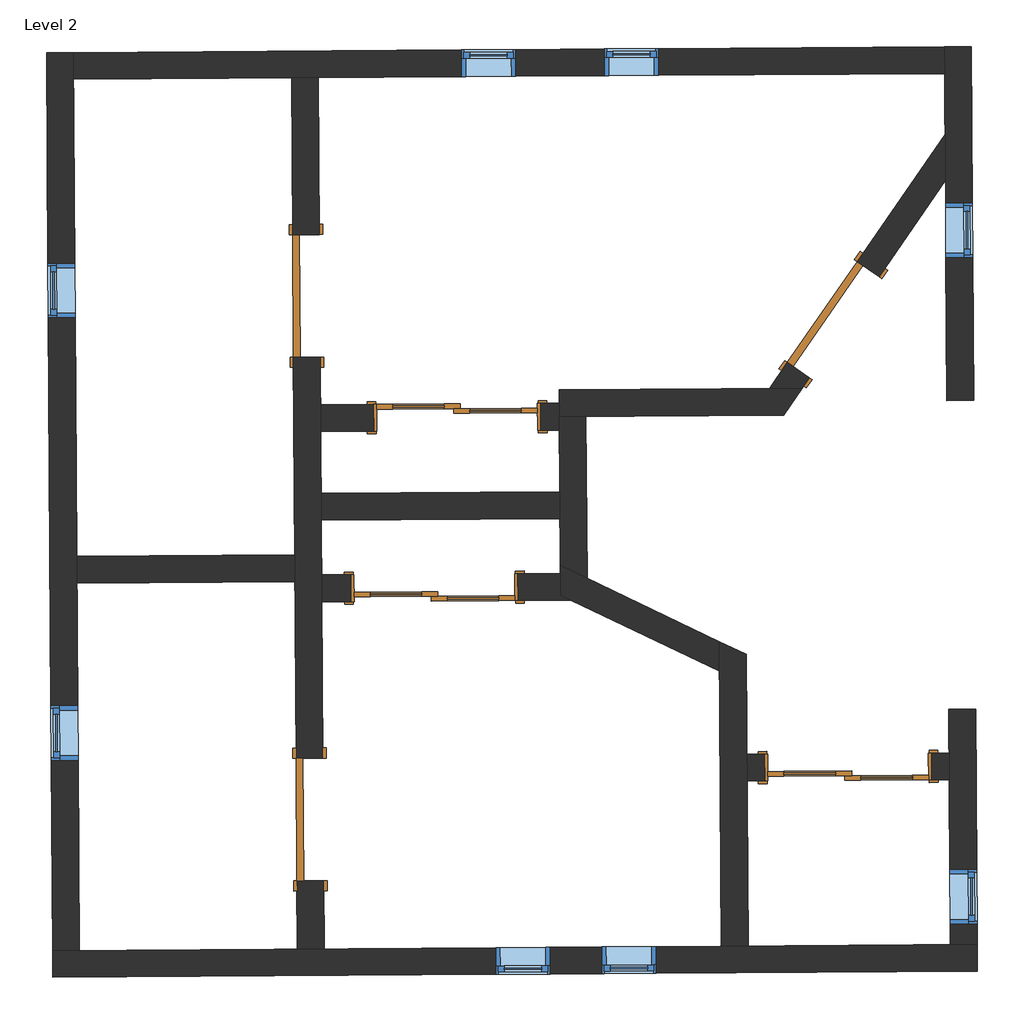
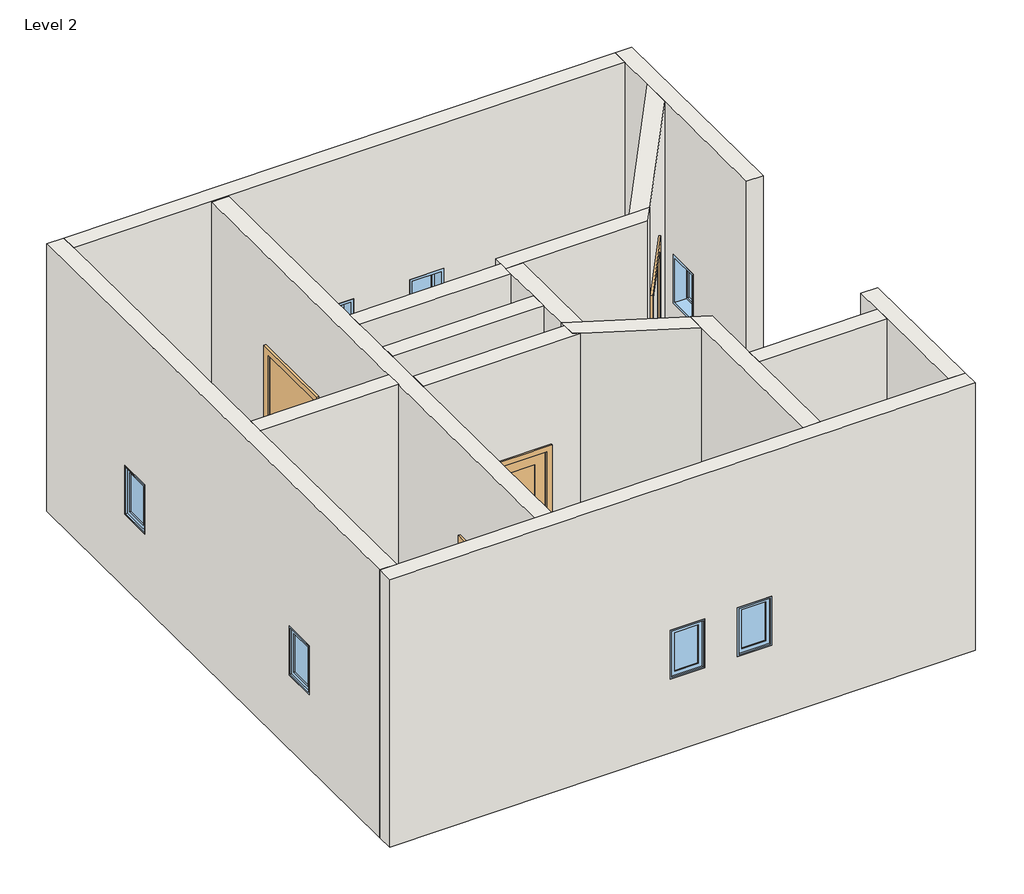
# One storey: 16 walls, 8 windows, 6 doors.
"""IFC4 building model written with IfcOpenShell, lengths in millimetres."""

import ifcopenshell
import ifcopenshell.guid

model = None  # the IFC model being written
_history = None  # IfcOwnerHistory: only IFC2X3 demands one
_inside = {}  # id of a spatial element -> (the spatial element, [elements in it])
_under = {}  # id of a project, library or spatial element -> (it, [spatial elements below it])
_declared = {}  # id of a project -> (the project, [libraries it declares])
_typed = {}  # id of a type object -> (the type object, [elements of that type])
_made_of = {}  # id of a material, layer set ... -> (it, [elements and type objects made of it])


def new_model(schema):
    """Start an empty IFC model of exactly this schema.

    Asked for "IFC4X3", IfcOpenShell would pick the latest addendum, in which some entities
    have other attributes; the version numbers below select the first issue.
    IFC2X3 requires an IfcOwnerHistory on every rooted entity: one is made here for all.
    """
    global model, _history
    if schema == "IFC4X3":
        model = ifcopenshell.file(schema_version=(4, 3, 0, 0))
    else:
        model = ifcopenshell.file(schema=schema)
    _inside.clear()
    _under.clear()
    _declared.clear()
    _typed.clear()
    _made_of.clear()
    _history = None
    if model.schema == "IFC2X3":
        org = make("IfcOrganization", Name="unknown")
        user = make(
            "IfcPersonAndOrganization",
            ThePerson=make("IfcPerson", FamilyName="unknown"),
            TheOrganization=org,
        )
        app = make(
            "IfcApplication",
            ApplicationDeveloper=org,
            Version="unknown",
            ApplicationFullName="unknown",
            ApplicationIdentifier="unknown",
        )
        _history = make(
            "IfcOwnerHistory",
            OwningUser=user,
            OwningApplication=app,
            ChangeAction="ADDED",
            CreationDate=0,
        )
    return model


def make(cls, **values):
    """One entity of the class cls with the attributes given. An attribute that is None is left unset."""
    return model.create_entity(
        cls, **{name: value for name, value in values.items() if value is not None}
    )


def rooted(cls, **values):
    """An entity with a GlobalId (a new one), such as an element, a storey or a relation."""
    return make(cls, GlobalId=ifcopenshell.guid.new(), OwnerHistory=_history, **values)


def si_unit(unit_type, name, prefix=None):
    """IfcSIUnit, for example si_unit("LENGTHUNIT", "METRE", prefix="MILLI")."""
    return make("IfcSIUnit", UnitType=unit_type, Prefix=prefix, Name=name)


def assignment(units):
    """IfcUnitAssignment: the units of a project."""
    return None if units is None else make("IfcUnitAssignment", Units=units)


def point(xyz):
    """IfcCartesianPoint."""
    return None if xyz is None else make("IfcCartesianPoint", Coordinates=xyz)


def direction(xyz):
    """IfcDirection."""
    return None if xyz is None else make("IfcDirection", DirectionRatios=xyz)


def frame(location, z_axis=None, x_axis=None):
    """IfcAxis2Placement3D, a coordinate frame: its origin and axes. An axis left out is left unset."""
    return make(
        "IfcAxis2Placement3D",
        Location=point(location),
        Axis=direction(z_axis),
        RefDirection=direction(x_axis),
    )


def origin():
    """The frame at (0, 0, 0) with its axes left unset."""
    return frame((0.0, 0.0, 0.0))


def origin_with_axes():
    """The frame at (0, 0, 0) with the z axis (0, 0, 1) and the x axis (1, 0, 0) written out."""
    return frame((0.0, 0.0, 0.0), z_axis=(0.0, 0.0, 1.0), x_axis=(1.0, 0.0, 0.0))


def place(relative_to, where):
    """IfcLocalPlacement: puts the frame where relative to a parent placement (None: the world)."""
    return make(
        "IfcLocalPlacement", PlacementRelTo=relative_to, RelativePlacement=where
    )


def context(
    kind, dimensions, precision=None, world=None, true_north=None, identifier=None
):
    """IfcGeometricRepresentationContext, for example the 3D "Model" context."""
    return make(
        "IfcGeometricRepresentationContext",
        ContextIdentifier=identifier,
        ContextType=kind,
        CoordinateSpaceDimension=dimensions,
        Precision=precision,
        WorldCoordinateSystem=world,
        TrueNorth=true_north,
    )


def project(units=None, contexts=None):
    """IfcProject with its units and contexts."""
    return rooted(
        "IfcProject",
        Name="project",
        RepresentationContexts=contexts,
        UnitsInContext=assignment(units),
    )


def spatial(cls, under=None, at=None, **own):
    """A site, building, storey or space (cls), placed at a placement, below another one or the project."""
    s = rooted(cls, ObjectPlacement=at, **own)
    if under is not None:
        _under.setdefault(under.id(), (under, []))[1].append(s)
    return s


def polyline(points):
    """IfcPolyline through the points."""
    return make("IfcPolyline", Points=[point(p) for p in points])


def outline(outer, holes=None, kind="AREA"):
    """IfcArbitraryClosedProfileDef: a profile drawn as a closed curve; with holes, ...WithVoids."""
    if holes is None:
        return make("IfcArbitraryClosedProfileDef", ProfileType=kind, OuterCurve=outer)
    return make(
        "IfcArbitraryProfileDefWithVoids",
        ProfileType=kind,
        OuterCurve=outer,
        InnerCurves=holes,
    )


def extrude(swept, where, along, depth):
    """IfcExtrudedAreaSolid: the profile swept, set in the frame where, extruded along a direction by depth."""
    return make(
        "IfcExtrudedAreaSolid",
        SweptArea=swept,
        Position=where,
        ExtrudedDirection=direction(along),
        Depth=depth,
    )


def faces_of(points, faces, orient=None, outer=None):
    """IfcFace entities. A face is a list of loops; a loop is a list of indices into points, from 0.

    orient and outer hold one flag for each loop. By default every Orientation is true, the
    first loop of a face is its IfcFaceOuterBound and the others are IfcFaceBound.
    """
    made = []
    for i, loops in enumerate(faces):
        bounds = []
        for j, loop in enumerate(loops):
            is_outer = j == 0 if outer is None else outer[i][j]
            bounds.append(
                make(
                    "IfcFaceOuterBound" if is_outer else "IfcFaceBound",
                    Bound=make("IfcPolyLoop", Polygon=[points[k] for k in loop]),
                    Orientation=True if orient is None else orient[i][j],
                )
            )
        made.append(make("IfcFace", Bounds=bounds))
    return made


def faceted_brep(points, faces, orient=None, outer=None, voids=None):
    """IfcFacetedBrep: a solid bounded by flat faces; with voids (closed shells), ...WithVoids."""
    shared = [point(p) for p in points]
    hull = make("IfcClosedShell", CfsFaces=faces_of(shared, faces, orient, outer))
    if voids is None:
        return make("IfcFacetedBrep", Outer=hull)
    return make(
        "IfcFacetedBrepWithVoids",
        Outer=hull,
        Voids=[
            make(cls, CfsFaces=faces_of(shared, fs, o, b)) for cls, fs, o, b in voids
        ],
    )


def shape(context_of_items, identifier, shape_type, items):
    """IfcShapeRepresentation: the items that make up one representation, for example the "Body"."""
    return make(
        "IfcShapeRepresentation",
        ContextOfItems=context_of_items,
        RepresentationIdentifier=identifier,
        RepresentationType=shape_type,
        Items=items,
    )


def source(mapping_origin, context_of_items, identifier, shape_type, items):
    """IfcRepresentationMap: a shape defined once, which mapped items show again and again."""
    return make(
        "IfcRepresentationMap",
        MappingOrigin=mapping_origin,
        MappedRepresentation=shape(context_of_items, identifier, shape_type, items),
    )


def transform(
    local_origin,
    x_axis=None,
    y_axis=None,
    z_axis=None,
    scale=None,
    scale2=None,
    scale3=None,
    uniform=True,
):
    """IfcCartesianTransformationOperator3D, or its non-uniform kind. x_axis, y_axis, z_axis: its Axis1, 2, 3."""
    if uniform:
        return make(
            "IfcCartesianTransformationOperator3D",
            Axis1=direction(x_axis),
            Axis2=direction(y_axis),
            LocalOrigin=point(local_origin),
            Scale=scale,
            Axis3=direction(z_axis),
        )
    return make(
        "IfcCartesianTransformationOperator3DnonUniform",
        Axis1=direction(x_axis),
        Axis2=direction(y_axis),
        LocalOrigin=point(local_origin),
        Scale=scale,
        Axis3=direction(z_axis),
        Scale2=scale2,
        Scale3=scale3,
    )


def mapped(mapping_source, mapping_target):
    """IfcMappedItem: shows the shape of a source again, moved by a transform."""
    return make(
        "IfcMappedItem", MappingSource=mapping_source, MappingTarget=mapping_target
    )


def made_of(thing, what):
    """Note that an element or type object is made of a material, layer set ...; save() writes the relation."""
    if what is not None:
        _made_of.setdefault(what.id(), (what, []))[1].append(thing)
    return thing


def element(
    cls,
    number,
    at=None,
    inside=None,
    cuts=None,
    type_object=None,
    material=None,
    context=None,
    identifier="Body",
    shape_type=None,
    held_by="IfcProductDefinitionShape",
    body=None,
    shapes=None,
    **own,
):
    """One element of the class cls, such as IfcWall. Its Tag is "e" and its number.

    at: its placement. inside: the storey or other place that contains it. cuts: it is an
    opening in that element (IfcRelVoidsElement). A single representation is given by context,
    identifier, shape_type and body (its items); several are given by shapes. held_by: the class
    of the entity that holds the representations. save() writes the other relations.
    """
    e = rooted(cls, Tag="e%d" % number, ObjectPlacement=at, **own)
    if body is not None:
        shapes = [shape(context, identifier, shape_type, body)]
    if shapes is not None:
        e.Representation = make(held_by, Representations=shapes)
    if inside is not None:
        _inside.setdefault(inside.id(), (inside, []))[1].append(e)
    if cuts is not None:
        rooted(
            "IfcRelVoidsElement", RelatingBuildingElement=cuts, RelatedOpeningElement=e
        )
    if type_object is not None:
        _typed.setdefault(type_object.id(), (type_object, []))[1].append(e)
    return made_of(e, material)


def aggregate(whole, parts):
    """IfcRelAggregates: a whole, such as a stair, and the parts it consists of."""
    return rooted("IfcRelAggregates", RelatingObject=whole, RelatedObjects=parts)


def save(model, path):
    """Write the relations noted so far, then the file.

    IfcRelAggregates (storeys below a building ...), IfcRelContainedInSpatialStructure (elements
    in a storey), IfcRelDefinesByType, IfcRelAssociatesMaterial and IfcRelDeclares: one each for
    every whole, place, type object, material and project.
    """
    for whole, parts in _under.values():
        aggregate(whole, parts)
    for where, things in _inside.values():
        rooted(
            "IfcRelContainedInSpatialStructure",
            RelatedElements=things,
            RelatingStructure=where,
        )
    for kind, things in _typed.values():
        rooted("IfcRelDefinesByType", RelatedObjects=things, RelatingType=kind)
    for what, things in _made_of.values():
        rooted("IfcRelAssociatesMaterial", RelatedObjects=things, RelatingMaterial=what)
    for by, libraries in _declared.values():
        rooted("IfcRelDeclares", RelatingContext=by, RelatedDefinitions=libraries)
    model.write(path)


def m_door_interior_double_sliding_2_panel_wood_1200_x_2000mm_2523b4d6(model_context):
    return source(origin(), model_context, "Body", "SweptSolid", [
        extrude(outline(polyline([(480.0, 38.4916667), (94.6, 38.4916667), (94.6, 50.1583333), (480.0, 50.1583333), (480.0, 38.4916667)])), frame((0.0, 0.0, 1014.4), z_axis=(0.0, 0.0, 1.0), x_axis=(1.0, 0.0, 0.0)), (0.0, 0.0, 1.0), 865.6),
        extrude(outline(polyline([(480.0, 38.4916667), (94.6, 38.4916667), (94.6, 50.1583333), (480.0, 50.1583333), (480.0, 38.4916667)])), frame((0.0, 0.0, 230.0), z_axis=(0.0, 0.0, 1.0), x_axis=(1.0, 0.0, 0.0)), (0.0, 0.0, 1.0), 584.4),
        extrude(outline(polyline([(2000.0, -25.4), (0.0, -25.4), (0.0, 600.0), (2000.0, 600.0), (2000.0, -25.4)]), holes=[polyline([(1880.0, 94.6), (1880.0, 480.0), (1014.4, 480.0), (1014.4, 94.6), (1880.0, 94.6)]), polyline([(814.4, 94.6), (814.4, 480.0), (230.0, 480.0), (230.0, 94.6), (814.4, 94.6)])]), frame((0.0, 26.825, 0.0), z_axis=(0.0, 1.0, 0.0), x_axis=(0.0, 0.0, 1.0)), (0.0, 0.0, 1.0), 35.0),
        extrude(outline(polyline([(-94.6, 73.4916667), (-480.0, 73.4916667), (-480.0, 85.1583333), (-94.6, 85.1583333), (-94.6, 73.4916667)])), frame((0.0, 0.0, 1014.4), z_axis=(0.0, 0.0, 1.0), x_axis=(1.0, 0.0, 0.0)), (0.0, 0.0, 1.0), 865.6),
        extrude(outline(polyline([(-94.6, 73.4916667), (-480.0, 73.4916667), (-480.0, 85.1583333), (-94.6, 85.1583333), (-94.6, 73.4916667)])), frame((0.0, 0.0, 230.0), z_axis=(0.0, 0.0, 1.0), x_axis=(1.0, 0.0, 0.0)), (0.0, 0.0, 1.0), 584.4),
        extrude(outline(polyline([(2000.0, -600.0), (0.0, -600.0), (0.0, 25.4), (2000.0, 25.4), (2000.0, -600.0)]), holes=[polyline([(1880.0, -480.0), (1880.0, -94.6), (1014.4, -94.6), (1014.4, -480.0), (1880.0, -480.0)]), polyline([(814.4, -480.0), (814.4, -94.6), (230.0, -94.6), (230.0, -480.0), (814.4, -480.0)])]), frame((0.0, 61.825, 0.0), z_axis=(0.0, 1.0, 0.0), x_axis=(0.0, 0.0, 1.0)), (0.0, 0.0, 1.0), 35.0),
        extrude(outline(polyline([(0.0, 600.0), (0.0, 625.0), (2025.0, 625.0), (2025.0, -625.0), (0.0, -625.0), (0.0, -600.0), (2000.0, -600.0), (2000.0, 600.0), (0.0, 600.0)])), frame((0.0, -103.175, 0.0), z_axis=(0.0, 1.0, 0.0), x_axis=(0.0, 0.0, 1.0)), (0.0, 0.0, 1.0), 200.0),
        extrude(outline(polyline([(0.0, 606.35), (0.0, 671.35), (2071.35, 671.35), (2071.35, -671.35), (0.0, -671.35), (0.0, -606.35), (2006.35, -606.35), (2006.35, 606.35), (0.0, 606.35)])), frame((0.0, -123.175, 0.0), z_axis=(0.0, 1.0, 0.0), x_axis=(0.0, 0.0, 1.0)), (0.0, 0.0, 1.0), 20.0),
        extrude(outline(polyline([(0.0, 606.35), (0.0, 671.35), (2071.35, 671.35), (2071.35, -671.35), (0.0, -671.35), (0.0, -606.35), (2006.35, -606.35), (2006.35, 606.35), (0.0, 606.35)])), frame((0.0, 96.825, 0.0), z_axis=(0.0, 1.0, 0.0), x_axis=(0.0, 0.0, 1.0)), (0.0, 0.0, 1.0), 20.0),
    ])


def m_single_flush_0915_x_2134mm_6a9e8738(model_context):
    return source(origin(), model_context, "Body", "SweptSolid", [
        extrude(outline(polyline([(2210.0, -533.5), (0.0, -533.5), (0.0, -457.5), (2134.0, -457.5), (2134.0, 457.5), (0.0, 457.5), (0.0, 533.5), (2210.0, 533.5), (2210.0, -533.5)])), frame((0.0, 100.0, 0.0), z_axis=(0.0, 1.0, 0.0), x_axis=(0.0, 0.0, 1.0)), (0.0, 0.0, 1.0), 25.0),
        extrude(outline(polyline([(2210.0, 533.5), (2210.0, -533.5), (0.0, -533.5), (0.0, -457.5), (2134.0, -457.5), (2134.0, 457.5), (0.0, 457.5), (0.0, 533.5), (2210.0, 533.5)])), frame((0.0, -125.0, 0.0), z_axis=(0.0, 1.0, 0.0), x_axis=(0.0, 0.0, 1.0)), (0.0, 0.0, 1.0), 25.0),
        extrude(outline(polyline([(457.5, 49.0), (-457.5, 49.0), (-457.5, 100.0), (457.5, 100.0), (457.5, 49.0)])), origin_with_axes(), (0.0, 0.0, 1.0), 2134.0),
    ])


def m_single_flush_0915_x_2134mm_727434cd(model_context):
    return source(origin(), model_context, "Body", "SweptSolid", [
        extrude(outline(polyline([(2210.0, -533.5), (0.0, -533.5), (0.0, -457.5), (2134.0, -457.5), (2134.0, 457.5), (0.0, 457.5), (0.0, 533.5), (2210.0, 533.5), (2210.0, -533.5)])), frame((0.0, -125.0, 0.0), z_axis=(0.0, 1.0, 0.0), x_axis=(0.0, 0.0, 1.0)), (0.0, 0.0, 1.0), 25.0),
        extrude(outline(polyline([(2210.0, 533.5), (2210.0, -533.5), (0.0, -533.5), (0.0, -457.5), (2134.0, -457.5), (2134.0, 457.5), (0.0, 457.5), (0.0, 533.5), (2210.0, 533.5)])), frame((0.0, 100.0, 0.0), z_axis=(0.0, 1.0, 0.0), x_axis=(0.0, 0.0, 1.0)), (0.0, 0.0, 1.0), 25.0),
        extrude(outline(polyline([(457.5, -49.0), (457.5, -100.0), (-457.5, -100.0), (-457.5, -49.0), (457.5, -49.0)])), origin_with_axes(), (0.0, 0.0, 1.0), 2134.0),
    ])


def m_fixed_0406_x_0610mm_8205b201(model_context):
    return source(origin(), model_context, "Body", "SweptSolid", [
        extrude(outline(polyline([(-140.0, 78.0), (140.0, 78.0), (140.0, 66.0), (-140.0, 66.0), (-140.0, 78.0)])), frame((0.0, 0.0, 978.0), z_axis=(0.0, 0.0, 1.0), x_axis=(1.0, 0.0, 0.0)), (0.0, 0.0, 1.0), 484.0),
        extrude(outline(polyline([(1506.0, -184.0), (934.0, -184.0), (934.0, 184.0), (1506.0, 184.0), (1506.0, -184.0)]), holes=[polyline([(1462.0, -140.0), (1462.0, 140.0), (978.0, 140.0), (978.0, -140.0), (1462.0, -140.0)])]), frame((0.0, 50.0, 0.0), z_axis=(0.0, 1.0, 0.0), x_axis=(0.0, 0.0, 1.0)), (0.0, 0.0, 1.0), 44.0),
        extrude(outline(polyline([(1525.0, -203.0), (915.0, -203.0), (915.0, 203.0), (1525.0, 203.0), (1525.0, -203.0)]), holes=[polyline([(1506.0, -184.0), (1506.0, 184.0), (934.0, 184.0), (934.0, -184.0), (1506.0, -184.0)])]), frame((0.0, 50.0, 0.0), z_axis=(0.0, 1.0, 0.0), x_axis=(0.0, 0.0, 1.0)), (0.0, 0.0, 1.0), 63.0),
        extrude(outline(polyline([(1525.0, -203.0), (915.0, -203.0), (915.0, 203.0), (1525.0, 203.0), (1525.0, -203.0)]), holes=[polyline([(1493.0, -171.0), (1493.0, 171.0), (947.0, 171.0), (947.0, -171.0), (1493.0, -171.0)])]), frame((0.0, -87.0, 0.0), z_axis=(0.0, 1.0, 0.0), x_axis=(0.0, 0.0, 1.0)), (0.0, 0.0, 1.0), 137.0),
    ])


model = new_model("IFC4")

# Units and contexts
model_context = context("Model", 3, world=origin())
ifc_project = project(units=[si_unit("LENGTHUNIT", "METRE", prefix="MILLI")], contexts=[model_context])

# Site, building, storey
site = spatial("IfcSite", under=ifc_project)
building = spatial("IfcBuilding", under=site)
storey = spatial("IfcBuildingStorey", under=building, Name="Level 2", Elevation=3048.0)

# Doors
placement = place(None, origin())
m_door_interior_double_sliding_2_panel_wood_1200_x_2000mm_shape = m_door_interior_double_sliding_2_panel_wood_1200_x_2000mm_2523b4d6(model_context)
element("IfcDoor", 1, ObjectType="M_Door-Interior-Double-Sliding-2_Panel-Wood : 1200 x 2000mm", at=placement, inside=storey, context=model_context, shape_type="MappedRepresentation", body=[
    mapped(m_door_interior_double_sliding_2_panel_wood_1200_x_2000mm_shape, transform((-71556.4861073, -7431.0700017, 3048.0), x_axis=(0.9999777944135733, 0.006664133834601911, 0.0), y_axis=(-0.006664133834601911, 0.9999777944135733, 0.0), z_axis=(0.0, 0.0, 1.0))),
])
element("IfcDoor", 2, ObjectType="M_Door-Interior-Double-Sliding-2_Panel-Wood : 1200 x 2000mm", at=placement, inside=storey, context=model_context, shape_type="MappedRepresentation", body=[
    mapped(m_door_interior_double_sliding_2_panel_wood_1200_x_2000mm_shape, transform((-71726.571382, -8709.3309667, 3048.0), x_axis=(-0.9999777944135733, -0.006664133834601911, 0.0), y_axis=(0.006664133834601911, -0.9999777944135733, 0.0), z_axis=(0.0, 0.0, 1.0))),
])
element("IfcDoor", 3, ObjectType="M_Door-Interior-Double-Sliding-2_Panel-Wood : 1200 x 2000mm", at=placement, inside=storey, context=model_context, shape_type="MappedRepresentation", body=[
    mapped(m_door_interior_double_sliding_2_panel_wood_1200_x_2000mm_shape, transform((-68636.4800539, -10048.7108484, 3048.0), x_axis=(-0.9999777944135733, -0.006664133834601911, 0.0), y_axis=(0.006664133834601911, -0.9999777944135733, 0.0), z_axis=(0.0, 0.0, 1.0))),
])
m_single_flush_0915_x_2134mm_shape = m_single_flush_0915_x_2134mm_6a9e8738(model_context)
element("IfcDoor", 4, ObjectType="M_Single-Flush : 0915 x 2134mm", at=placement, inside=storey, context=model_context, shape_type="MappedRepresentation", body=[
    mapped(m_single_flush_0915_x_2134mm_shape, transform((-68747.95097, -6705.2508945, 3048.0), x_axis=(0.5681047608958888, 0.8229562446736918, 0.0), y_axis=(-0.8229562446736918, 0.5681047608958888, 0.0), z_axis=(0.0, 0.0, 1.0))),
])
element("IfcDoor", 5, ObjectType="M_Single-Flush : 0915 x 2134mm", at=placement, inside=storey, context=model_context, shape_type="MappedRepresentation", body=[
    mapped(m_single_flush_0915_x_2134mm_shape, transform((-72681.7331306, -6527.4212039, 3048.0), x_axis=(-0.0066641338345986775, 0.9999777944135734, 0.0), y_axis=(-0.9999777944135734, -0.0066641338345986775, 0.0), z_axis=(0.0, 0.0, 1.0))),
])
m_single_flush_0915_x_2134mm_2_shape = m_single_flush_0915_x_2134mm_727434cd(model_context)
element("IfcDoor", 6, ObjectType="M_Single-Flush : 0915 x 2134mm", at=placement, inside=storey, context=model_context, shape_type="MappedRepresentation", body=[
    mapped(m_single_flush_0915_x_2134mm_2_shape, transform((-72655.6757177, -10437.4318493, 3048.0), x_axis=(0.0066641338345986775, -0.9999777944135734, 0.0), y_axis=(0.9999777944135734, 0.0066641338345986775, 0.0), z_axis=(0.0, 0.0, 1.0))),
])

# Walls
element("IfcWall", 7, ObjectType="Generic - 200mm", at=placement, inside=storey, context=model_context, shape_type="Brep", body=[
    faceted_brep([(-67672.5433459, -11371.0443197, 3048.0), (-67872.5389048, -11372.3771465, 3048.0), (-69382.7115618, -11382.4413627, 3048.0), (-69582.7071207, -11383.7741894, 3048.0), (-72549.2350537, -11403.5439676, 3048.0), (-72749.2306126, -11404.8767944, 3048.0), (-74377.9944441, -11415.7313355, 3048.0), (-74577.990003, -11417.0641623, 3048.0), (-74577.990003, -11417.0641623, 6372.225), (-74377.9944441, -11415.7313355, 6372.225), (-69582.7071207, -11383.7741894, 6372.225), (-69382.7115618, -11382.4413627, 6372.225), (-67872.5389048, -11372.3771465, 6372.225), (-67672.5433459, -11371.0443197, 6372.225), (-70862.9755949, -11392.3062593, 3963.0), (-70862.9755949, -11392.3062593, 4573.0), (-71268.9665794, -11395.0118977, 4573.0), (-71268.9665794, -11395.0118977, 3963.0), (-70071.3447219, -11387.0306081, 3963.0), (-70071.3447219, -11387.0306081, 4573.0), (-70477.3357065, -11389.7362464, 4573.0), (-70477.3357065, -11389.7362464, 3963.0), (-67671.2105191, -11571.0398786, 3048.0), (-67671.2105191, -11571.0398786, 6372.225), (-74576.6571762, -11617.0597212, 6372.225), (-74576.6571762, -11617.0597212, 3048.0), (-70861.6427681, -11592.3018182, 3963.0), (-71267.6337527, -11595.0074566, 3963.0), (-71267.6337527, -11595.0074566, 4573.0), (-70861.6427681, -11592.3018182, 4573.0), (-70070.0118952, -11587.026167, 3963.0), (-70476.0028797, -11589.7318053, 3963.0), (-70476.0028797, -11589.7318053, 4573.0), (-70070.0118952, -11587.026167, 4573.0)], [[[0, 1, 2, 3, 4, 5, 6, 7, 8, 9, 10, 11, 12, 13], [14, 15, 16, 17], [18, 19, 20, 21]], [[22, 23, 24, 25], [26, 27, 28, 29], [30, 31, 32, 33]], [[7, 6, 5, 4, 3, 2, 1, 0, 22, 25]], [[13, 12, 11, 10, 9, 8, 24, 23]], [[8, 7, 25, 24]], [[0, 13, 23, 22]], [[15, 14, 26, 29]], [[16, 15, 29, 28]], [[17, 16, 28, 27]], [[14, 17, 27, 26]], [[19, 18, 30, 33]], [[20, 19, 33, 32]], [[21, 20, 32, 31]], [[18, 21, 31, 30]]]),
])
element("IfcWall", 8, ObjectType="Generic - 200mm", at=placement, inside=storey, context=model_context, shape_type="Brep", body=[
    faceted_brep([(-74377.9944441, -11415.7313355, 3048.0), (-74396.2767952, -8672.3973113, 3048.0), (-74397.6096219, -8472.4017524, 3048.0), (-74421.3486332, -4910.2757962, 3048.0), (-74422.6814599, -4710.2802373, 3048.0), (-74422.6814599, -4710.2802373, 6372.225), (-74421.3486332, -4910.2757962, 6372.225), (-74397.6096219, -8472.4017524, 6372.225), (-74396.2767952, -8672.3973113, 6372.225), (-74377.9944441, -11415.7313355, 6372.225), (-74409.4904734, -6689.6362836, 3963.0), (-74409.4904734, -6689.6362836, 4573.0), (-74412.1961118, -6283.6452991, 4573.0), (-74412.1961118, -6283.6452991, 3963.0), (-74387.4654774, -9994.567951, 3963.0), (-74387.4654774, -9994.567951, 4573.0), (-74390.1711157, -9588.5769665, 4573.0), (-74390.1711157, -9588.5769665, 3963.0), (-74577.990003, -11417.0641623, 3048.0), (-74577.990003, -11417.0641623, 6372.225), (-74622.6770188, -4711.6130641, 6372.225), (-74622.6770188, -4711.6130641, 3048.0), (-74609.4860323, -6690.9691104, 3963.0), (-74612.1916706, -6284.9781258, 3963.0), (-74612.1916706, -6284.9781258, 4573.0), (-74609.4860323, -6690.9691104, 4573.0), (-74587.4610363, -9995.9007778, 3963.0), (-74590.1666746, -9589.9097933, 3963.0), (-74590.1666746, -9589.9097933, 4573.0), (-74587.4610363, -9995.9007778, 4573.0)], [[[0, 1, 2, 3, 4, 5, 6, 7, 8, 9], [10, 11, 12, 13], [14, 15, 16, 17]], [[18, 19, 20, 21], [22, 23, 24, 25], [26, 27, 28, 29]], [[4, 3, 2, 1, 0, 18, 21]], [[9, 8, 7, 6, 5, 20, 19]], [[0, 9, 19, 18]], [[5, 4, 21, 20]], [[11, 10, 22, 25]], [[12, 11, 25, 24]], [[13, 12, 24, 23]], [[10, 13, 23, 22]], [[15, 14, 26, 29]], [[16, 15, 29, 28]], [[17, 16, 28, 27]], [[14, 17, 27, 26]]]),
])
element("IfcWall", 9, ObjectType="Generic - 200mm", at=placement, inside=storey, context=model_context, shape_type="Brep", body=[
    faceted_brep([(-74421.3486332, -4910.2757962, 3048.0), (-72792.5848016, -4899.421255, 3048.0), (-72592.5892428, -4898.0884283, 3048.0), (-67915.8930938, -4866.9216071, 3048.0), (-67915.8930938, -4866.9216071, 6372.225), (-74421.3486332, -4910.2757962, 6372.225), (-70457.2366606, -4883.8578369, 3963.0), (-70457.2366606, -4883.8578369, 4573.0), (-70051.245676, -4881.1521985, 4573.0), (-70051.245676, -4881.1521985, 3963.0), (-71524.0129716, -4890.9671348, 3963.0), (-71524.0129716, -4890.9671348, 4573.0), (-71118.0219871, -4888.2614965, 4573.0), (-71118.0219871, -4888.2614965, 3963.0), (-74422.6814599, -4710.2802373, 3048.0), (-74422.6814599, -4710.2802373, 6372.225), (-67917.2259206, -4666.9260483, 6372.225), (-67917.2259206, -4666.9260483, 3048.0), (-70458.5694873, -4683.862278, 3963.0), (-70052.5785028, -4681.1566396, 3963.0), (-70052.5785028, -4681.1566396, 4573.0), (-70458.5694873, -4683.862278, 4573.0), (-71525.3457984, -4690.971576, 3963.0), (-71119.3548139, -4688.2659376, 3963.0), (-71119.3548139, -4688.2659376, 4573.0), (-71525.3457984, -4690.971576, 4573.0)], [[[0, 1, 2, 3, 4, 5], [6, 7, 8, 9], [10, 11, 12, 13]], [[14, 15, 16, 17], [18, 19, 20, 21], [22, 23, 24, 25]], [[3, 2, 1, 0, 14, 17]], [[5, 4, 16, 15]], [[0, 5, 15, 14]], [[7, 6, 18, 21]], [[8, 7, 21, 20]], [[9, 8, 20, 19]], [[6, 9, 19, 18]], [[11, 10, 22, 25]], [[12, 11, 25, 24]], [[13, 12, 24, 23]], [[10, 13, 23, 22]], [[4, 3, 17, 16]]]),
])
element("IfcWall", 10, ObjectType="Generic - 200mm", at=placement, inside=storey, context=model_context, shape_type="Brep", body=[
    faceted_brep([(-67917.2259206, -4666.9260483, 3048.0), (-67915.8930938, -4866.9216071, 3048.0), (-67912.8767245, -5319.5389284, 3048.0), (-67910.5530119, -5668.2205446, 3048.0), (-67899.6125812, -7309.8724158, 3048.0), (-67899.6125812, -7309.8724158, 6372.225), (-67910.5530119, -5668.2205446, 6372.225), (-67912.8767245, -5319.5389284, 6372.225), (-67915.8930938, -4866.9216071, 6372.225), (-67917.2259206, -4666.9260483, 6372.225), (-67909.4388634, -5835.4026295, 3963.0), (-67909.4388634, -5835.4026295, 4573.0), (-67906.733225, -6241.393614, 4573.0), (-67906.733225, -6241.393614, 3963.0), (-67717.2303617, -4665.5932215, 3048.0), (-67717.2303617, -4665.5932215, 6372.225), (-67699.6170223, -7308.539589, 6372.225), (-67699.6170223, -7308.539589, 3048.0), (-67709.4433045, -5834.0698027, 3963.0), (-67706.7376661, -6240.0607872, 3963.0), (-67706.7376661, -6240.0607872, 4573.0), (-67709.4433045, -5834.0698027, 4573.0)], [[[0, 1, 2, 3, 4, 5, 6, 7, 8, 9], [10, 11, 12, 13]], [[14, 15, 16, 17], [18, 19, 20, 21]], [[4, 3, 2, 1, 0, 14, 17]], [[5, 4, 17, 16]], [[9, 8, 7, 6, 5, 16, 15]], [[11, 10, 18, 21]], [[12, 11, 21, 20]], [[13, 12, 20, 19]], [[10, 13, 19, 18]], [[0, 9, 15, 14]]]),
])
element("IfcWall", 11, ObjectType="Generic - 200mm", at=placement, inside=storey, context=model_context, shape_type="Brep", body=[
    faceted_brep([(-67672.5433459, -11371.0443197, 3048.0), (-67684.2508882, -9614.2845298, 3048.0), (-67684.2508882, -9614.2845298, 6372.225), (-67672.5433459, -11371.0443197, 6372.225), (-67676.2765937, -10810.8567593, 3963.0), (-67673.5709553, -11216.8477438, 3963.0), (-67673.5709553, -11216.8477438, 4573.0), (-67676.2765937, -10810.8567593, 4573.0), (-67872.5389048, -11372.3771465, 3048.0), (-67872.5389048, -11372.3771465, 6372.225), (-67880.7484706, -10140.5015903, 6372.225), (-67882.0812974, -9940.5060314, 6372.225), (-67884.2464471, -9615.6173566, 6372.225), (-67884.2464471, -9615.6173566, 3048.0), (-67882.0812974, -9940.5060314, 3048.0), (-67880.7484706, -10140.5015903, 3048.0), (-67876.2721525, -10812.189586, 3963.0), (-67876.2721525, -10812.189586, 4573.0), (-67873.5665142, -11218.1805706, 4573.0), (-67873.5665142, -11218.1805706, 3963.0)], [[[0, 1, 2, 3], [4, 5, 6, 7]], [[8, 9, 10, 11, 12, 13, 14, 15], [16, 17, 18, 19]], [[1, 0, 8, 15, 14, 13]], [[2, 1, 13, 12]], [[3, 2, 12, 11, 10, 9]], [[0, 3, 9, 8]], [[17, 16, 4, 7]], [[18, 17, 7, 6]], [[19, 18, 6, 5]], [[16, 19, 5, 4]]]),
])
element("IfcWall", 12, ObjectType="Generic - 200mm", at=placement, inside=storey, context=model_context, shape_type="Brep", body=[
    faceted_brep([(-72752.6246559, -10895.5881037, 5182.0), (-72752.6246559, -10895.5881037, 3048.0), (-72749.2306126, -11404.8767944, 3048.0), (-72749.2306126, -11404.8767944, 6363.9898437), (-72792.5848016, -4899.421255, 6363.9898437), (-72792.5848016, -4899.421255, 3048.0), (-72784.7797512, -6070.5977763, 3048.0), (-72784.7797512, -6070.5977763, 5182.0), (-72778.6820688, -6985.5774582, 5182.0), (-72778.6820688, -6985.5774582, 3048.0), (-72768.8457904, -8461.5472112, 3048.0), (-72767.5129636, -8661.5427701, 3048.0), (-72758.7223384, -9980.6084218, 3048.0), (-72758.7223384, -9980.6084218, 5182.0), (-72549.2350537, -11403.5439676, 3048.0), (-72552.629097, -10894.2552769, 3048.0), (-72552.629097, -10894.2552769, 5182.0), (-72558.7267795, -9979.275595, 5182.0), (-72558.7267795, -9979.275595, 3048.0), (-72566.5074612, -8811.7556875, 3048.0), (-72567.840288, -8611.7601286, 3048.0), (-72570.5642467, -8203.0200957, 3048.0), (-72571.8970735, -8003.0245368, 3048.0), (-72574.9759033, -7541.0347958, 3048.0), (-72576.3087301, -7341.0392369, 3048.0), (-72578.6865099, -6984.2446314, 3048.0), (-72578.6865099, -6984.2446314, 5182.0), (-72584.7841924, -6069.2649495, 5182.0), (-72584.7841924, -6069.2649495, 3048.0), (-72592.5892428, -4898.0884283, 3048.0), (-72592.5892428, -4898.0884283, 6363.9898437), (-72549.2350537, -11403.5439676, 6363.9898437)], [[[0, 1, 2, 3, 4, 5, 6, 7, 8, 9, 10, 11, 12, 13]], [[14, 15, 16, 17, 18, 19, 20, 21, 22, 23, 24, 25, 26, 27, 28, 29, 30, 31]], [[3, 2, 14, 31]], [[5, 4, 30, 29]], [[7, 6, 28, 27]], [[8, 7, 27, 26]], [[9, 8, 26, 25]], [[16, 15, 1, 0]], [[17, 16, 0, 13]], [[18, 17, 13, 12]], [[29, 28, 6, 5]], [[2, 1, 15, 14]], [[12, 11, 10, 9, 25, 24, 23, 22, 21, 20, 19, 18]], [[4, 3, 31, 30]]]),
])
element("IfcWall", 13, ObjectType="Generic - 200mm", at=placement, inside=storey, context=model_context, shape_type="Brep", body=[
    faceted_brep([(-70794.4818693, -7429.1668612, 3048.0), (-70594.4863104, -7427.8340344, 3048.0), (-69118.4623821, -7417.997395, 3048.0), (-69118.4623821, -7417.997395, 6372.225), (-70594.4863104, -7427.8340344, 6372.225), (-70794.4818693, -7429.1668612, 6372.225), (-70795.8146961, -7229.1713023, 3048.0), (-70795.8146961, -7229.1713023, 6372.225), (-69223.906307, -7218.6956618, 6372.225), (-68979.7568109, -7217.0685807, 6372.225), (-68979.7568109, -7217.0685807, 3048.0), (-69223.906307, -7218.6956618, 3048.0), (-70795.1482827, -7329.1690817, 3048.0), (-70795.1482827, -7329.1690817, 6372.225)], [[[0, 1, 2, 3, 4, 5]], [[6, 7, 8, 9, 10, 11]], [[2, 1, 0, 12, 6, 11, 10]], [[5, 4, 3, 9, 8, 7, 13]], [[3, 2, 10, 9]], [[0, 5, 13, 7, 6, 12]]]),
])
element("IfcWall", 14, ObjectType="Generic - 200mm", at=placement, inside=storey, context=model_context, shape_type="Brep", body=[
    faceted_brep([(-68405.7474175, -6385.5588886, 5182.0), (-68405.7474175, -6385.5588886, 3048.0), (-67910.5530119, -5668.2205446, 3048.0), (-67910.5530119, -5668.2205446, 6372.225), (-68979.7568109, -7217.0685807, 6372.225), (-68979.7568109, -7217.0685807, 3048.0), (-68925.5632737, -7138.5638525, 3048.0), (-68925.5632737, -7138.5638525, 5182.0), (-67912.8767245, -5319.5389284, 3048.0), (-68570.3386664, -6271.9379364, 3048.0), (-68570.3386664, -6271.9379364, 5182.0), (-69090.1545226, -7024.9429003, 5182.0), (-69090.1545226, -7024.9429003, 3048.0), (-69223.906307, -7218.6956618, 3048.0), (-69223.906307, -7218.6956618, 6372.225), (-67912.8767245, -5319.5389284, 6372.225)], [[[0, 1, 2, 3, 4, 5, 6, 7]], [[8, 9, 10, 11, 12, 13, 14, 15]], [[6, 5, 13, 12]], [[2, 1, 9, 8]], [[4, 3, 15, 14]], [[5, 4, 14, 13]], [[3, 2, 8, 15]], [[10, 9, 1, 0]], [[11, 10, 0, 7]], [[12, 11, 7, 6]]]),
])
element("IfcWall", 15, ObjectType="Generic - 200mm", at=placement, inside=storey, context=model_context, shape_type="Brep", body=[
    faceted_brep([(-69597.8683674, -9108.7733463, 3048.0), (-69596.3862055, -9331.1771945, 3048.0), (-69582.7071207, -11383.7741894, 3048.0), (-69582.7071207, -11383.7741894, 6372.225), (-69596.3862055, -9331.1771945, 6372.225), (-69597.8683674, -9108.7733463, 6372.225), (-69397.2244438, -9204.7300262, 3048.0), (-69397.2244438, -9204.7300262, 6372.225), (-69392.2539544, -9950.5702476, 6372.225), (-69390.9211276, -10150.5658065, 6372.225), (-69382.7115618, -11382.4413627, 6372.225), (-69382.7115618, -11382.4413627, 3048.0), (-69390.9211276, -10150.5658065, 3048.0), (-69392.2539544, -9950.5702476, 3048.0)], [[[0, 1, 2, 3, 4, 5]], [[6, 7, 8, 9, 10, 11, 12, 13]], [[2, 1, 0, 6, 13, 12, 11]], [[5, 4, 3, 10, 9, 8, 7]], [[3, 2, 11, 10]], [[0, 5, 7, 6]]]),
])
element("IfcWall", 16, ObjectType="Generic - 200mm", at=placement, inside=storey, context=model_context, shape_type="Brep", body=[
    faceted_brep([(-70785.5965285, -8762.4449236, 3048.0), (-70708.3813089, -8799.3726112, 3048.0), (-69596.3862055, -9331.1771945, 3048.0), (-69596.3862055, -9331.1771945, 6372.225), (-70708.3813089, -8799.3726112, 6372.225), (-70785.5965285, -8762.4449236, 6372.225), (-70787.0786905, -8540.0410755, 3048.0), (-70787.0786905, -8540.0410755, 6372.225), (-70586.4347669, -8635.9977554, 6372.225), (-69597.8683674, -9108.7733463, 6372.225), (-69597.8683674, -9108.7733463, 3048.0), (-70586.4347669, -8635.9977554, 3048.0), (-70786.6798405, -8599.8899734, 3048.0), (-70786.6798405, -8599.8899734, 6372.225)], [[[0, 1, 2, 3, 4, 5]], [[6, 7, 8, 9, 10, 11]], [[2, 1, 0, 12, 6, 11, 10]], [[5, 4, 3, 9, 8, 7, 13]], [[3, 2, 10, 9]], [[0, 5, 13, 7, 6, 12]]]),
])
element("IfcWall", 17, ObjectType="Generic - 200mm", at=placement, inside=storey, context=model_context, shape_type="Brep", body=[
    faceted_brep([(-70794.4818693, -7429.1668612, 3048.0), (-70793.8154559, -7529.1646406, 3048.0), (-70790.7366261, -7991.1543816, 3048.0), (-70789.4037993, -8191.1499405, 3048.0), (-70787.0786905, -8540.0410755, 3048.0), (-70787.0786905, -8540.0410755, 6372.225), (-70789.4037993, -8191.1499405, 6372.225), (-70790.7366261, -7991.1543816, 6372.225), (-70793.8154559, -7529.1646406, 6372.225), (-70794.4818693, -7429.1668612, 6372.225), (-70594.4863104, -7427.8340344, 3048.0), (-70594.4863104, -7427.8340344, 6372.225), (-70586.4347669, -8635.9977554, 6372.225), (-70586.4347669, -8635.9977554, 3048.0)], [[[0, 1, 2, 3, 4, 5, 6, 7, 8, 9]], [[10, 11, 12, 13]], [[4, 3, 2, 1, 0, 10, 13]], [[9, 8, 7, 6, 5, 12, 11]], [[0, 9, 11, 10]], [[5, 4, 13, 12]]]),
])
element("IfcWall", 18, ObjectType="Generic - 200mm", at=placement, inside=storey, context=model_context, shape_type="SweptSolid", body=[
    extrude(outline(polyline([(-74397.6096219, -8472.4017524), (-72768.8457904, -8461.5472112), (-72767.5129636, -8661.5427701), (-74396.2767952, -8672.3973113), (-74397.6096219, -8472.4017524)])), frame((0.0, 0.0, 3048.0), z_axis=(0.0, 0.0, 1.0), x_axis=(1.0, 0.0, 0.0)), (0.0, 0.0, 1.0), 3324.225),
])
element("IfcWall", 19, ObjectType="Generic - 200mm", at=placement, inside=storey, context=model_context, shape_type="Brep", body=[
    faceted_brep([(-72576.3087301, -7341.0392369, 6372.225), (-70795.1482827, -7329.1690817, 6372.225), (-70795.1482827, -7329.1690817, 3048.0), (-70932.1452405, -7330.0820681, 3048.0), (-70932.1452405, -7330.0820681, 5073.0), (-72182.1174835, -7338.4122354, 5073.0), (-72182.1174835, -7338.4122354, 3048.0), (-72576.3087301, -7341.0392369, 3048.0), (-70793.8154559, -7529.1646406, 6372.225), (-72574.9759033, -7541.0347958, 6372.225), (-72574.9759033, -7541.0347958, 3048.0), (-72180.7846568, -7538.4077942, 3048.0), (-72180.7846568, -7538.4077942, 5073.0), (-70930.8124138, -7530.0776269, 5073.0), (-70930.8124138, -7530.0776269, 3048.0), (-70793.8154559, -7529.1646406, 3048.0), (-70794.4818693, -7429.1668612, 3048.0), (-70794.4818693, -7429.1668612, 6372.225)], [[[0, 1, 2, 3, 4, 5, 6, 7]], [[8, 9, 10, 11, 12, 13, 14, 15]], [[2, 16, 15, 14, 3]], [[10, 7, 6, 11]], [[1, 0, 9, 8, 17]], [[0, 7, 10, 9]], [[2, 1, 17, 8, 15, 16]], [[13, 4, 3, 14]], [[4, 13, 12, 5]], [[5, 12, 11, 6]]]),
])
element("IfcWall", 20, ObjectType="Generic - 200mm", at=placement, inside=storey, context=model_context, shape_type="Brep", body=[
    faceted_brep([(-72567.840288, -8611.7601286, 6372.225), (-70786.6798405, -8599.8899734, 6372.225), (-70786.6798405, -8599.8899734, 3048.0), (-71102.2728325, -8601.9931741, 3048.0), (-71102.2728325, -8601.9931741, 5073.0), (-72352.2450755, -8610.3233414, 5073.0), (-72352.2450755, -8610.3233414, 3048.0), (-72567.840288, -8611.7601286, 3048.0), (-70708.3813089, -8799.3726112, 6372.225), (-72566.5074612, -8811.7556875, 6372.225), (-72566.5074612, -8811.7556875, 3048.0), (-72350.9122487, -8810.3189003, 3048.0), (-72350.9122487, -8810.3189003, 5073.0), (-71100.9400057, -8801.988733, 5073.0), (-71100.9400057, -8801.988733, 3048.0), (-70708.3813089, -8799.3726112, 3048.0), (-70785.5965285, -8762.4449236, 3048.0), (-70785.5965285, -8762.4449236, 6372.225)], [[[0, 1, 2, 3, 4, 5, 6, 7]], [[8, 9, 10, 11, 12, 13, 14, 15]], [[2, 16, 15, 14, 3]], [[10, 7, 6, 11]], [[1, 0, 9, 8, 17]], [[2, 1, 17, 16]], [[8, 15, 16, 17]], [[0, 7, 10, 9]], [[5, 12, 11, 6]], [[12, 5, 4, 13]], [[13, 4, 3, 14]]]),
])
element("IfcWall", 21, ObjectType="Generic - 200mm", at=placement, inside=storey, context=model_context, shape_type="SweptSolid", body=[
    extrude(outline(polyline([(-72571.8970735, -8003.0245368), (-70790.7366261, -7991.1543816), (-70789.4037993, -8191.1499405), (-72570.5642467, -8203.0200957), (-72571.8970735, -8003.0245368)])), frame((0.0, 0.0, 3048.0), z_axis=(0.0, 0.0, 1.0), x_axis=(1.0, 0.0, 0.0)), (0.0, 0.0, 1.0), 3324.225),
])
element("IfcWall", 22, ObjectType="Generic - 200mm", at=placement, inside=storey, context=model_context, shape_type="SweptSolid", body=[
    extrude(outline(polyline([(0.0, -3324.225), (-1510.206192, -3324.225), (-1510.206192, 0.0), (-1380.103096, 0.0), (-1380.103096, -2025.0), (-130.103096, -2025.0), (-130.103096, 0.0), (0.0, 0.0), (0.0, -3324.225)])), frame((-67880.7484706, -10140.5015903, 3048.0), z_axis=(-0.006664133834601911, 0.9999777944135733, 0.0), x_axis=(0.9999777944135733, 0.006664133834601911, 0.0)), (0.0, 0.0, 1.0), 200.0),
])

# Windows
m_fixed_0406_x_0610mm_shape = m_fixed_0406_x_0610mm_8205b201(model_context)
element("IfcWindow", 23, ObjectType="M_Fixed : 0406 x 0610mm", at=placement, inside=storey, context=model_context, shape_type="MappedRepresentation", body=[
    mapped(m_fixed_0406_x_0610mm_shape, transform((-67787.9212653, -11014.6052987, 3048.0), x_axis=(0.006664133834598511, -0.9999777944135734, 0.0), y_axis=(0.9999777944135734, 0.006664133834598511, 0.0), z_axis=(0.0, 0.0, 1.0))),
])
element("IfcWindow", 24, ObjectType="M_Fixed : 0406 x 0610mm", at=placement, inside=storey, context=model_context, shape_type="MappedRepresentation", body=[
    mapped(m_fixed_0406_x_0610mm_shape, transform((-67821.0879761, -6037.8183421, 3048.0), x_axis=(0.006664133834604721, -0.9999777944135733, 0.0), y_axis=(0.9999777944135733, 0.006664133834604721, 0.0), z_axis=(0.0, 0.0, 1.0))),
])
element("IfcWindow", 25, ObjectType="M_Fixed : 0406 x 0610mm", at=placement, inside=storey, context=model_context, shape_type="MappedRepresentation", body=[
    mapped(m_fixed_0406_x_0610mm_shape, transform((-74497.8413607, -6487.220571, 3048.0), x_axis=(-0.006664133834601911, 0.9999777944135733, 0.0), y_axis=(-0.9999777944135733, -0.006664133834601911, 0.0), z_axis=(0.0, 0.0, 1.0))),
])
element("IfcWindow", 26, ObjectType="M_Fixed : 0406 x 0610mm", at=placement, inside=storey, context=model_context, shape_type="MappedRepresentation", body=[
    mapped(m_fixed_0406_x_0610mm_shape, transform((-74475.8163647, -9792.1522384, 3048.0), x_axis=(-0.006664133834601911, 0.9999777944135733, 0.0), y_axis=(-0.9999777944135733, -0.006664133834601911, 0.0), z_axis=(0.0, 0.0, 1.0))),
])
element("IfcWindow", 27, ObjectType="M_Fixed : 0406 x 0610mm", at=placement, inside=storey, context=model_context, shape_type="MappedRepresentation", body=[
    mapped(m_fixed_0406_x_0610mm_shape, transform((-70254.8209479, -4795.5069496, 3048.0), x_axis=(0.9999777944135733, 0.006664133834600627, 0.0), y_axis=(-0.006664133834600627, 0.9999777944135733, 0.0), z_axis=(0.0, 0.0, 1.0))),
])
element("IfcWindow", 28, ObjectType="M_Fixed : 0406 x 0610mm", at=placement, inside=storey, context=model_context, shape_type="MappedRepresentation", body=[
    mapped(m_fixed_0406_x_0610mm_shape, transform((-71321.597259, -4802.6162476, 3048.0), x_axis=(0.9999777944135733, 0.006664133834600627, 0.0), y_axis=(-0.006664133834600627, 0.9999777944135733, 0.0), z_axis=(0.0, 0.0, 1.0))),
])
element("IfcWindow", 29, ObjectType="M_Fixed : 0406 x 0610mm", at=placement, inside=storey, context=model_context, shape_type="MappedRepresentation", body=[
    mapped(m_fixed_0406_x_0610mm_shape, transform((-71065.3913075, -11480.6571466, 3048.0), x_axis=(-0.9999777944135733, -0.006664133834601911, 0.0), y_axis=(0.006664133834601911, -0.9999777944135733, 0.0), z_axis=(0.0, 0.0, 1.0))),
])
element("IfcWindow", 30, ObjectType="M_Fixed : 0406 x 0610mm", at=placement, inside=storey, context=model_context, shape_type="MappedRepresentation", body=[
    mapped(m_fixed_0406_x_0610mm_shape, transform((-70273.7604345, -11475.3814954, 3048.0), x_axis=(-0.9999777944135733, -0.006664133834601911, 0.0), y_axis=(0.006664133834601911, -0.9999777944135733, 0.0), z_axis=(0.0, 0.0, 1.0))),
])

save(model, "model.ifc")

# Revit data of these elements
# Project information
#   Project Issue Date = "Issue Date"
#   Project Status = "Project Status"
#   Client Name = "Owner"
#   Project Address = "Enter address here"
#   Project Name = "Project Name"
#   Project Number = "Project Number"
# Type "M_Door-Interior-Double-Sliding-2_Panel-Wood : 1200 x 2000mm"
#   Type Mark = "23"
#   Assembly Code = "C1020300"
#   Analytic Construction = "Wooden"
#   Top Rail = 0' - 4.72441"
#   Thickness = 0' - 1.37795"
#   Thermal Resistance (R) = 0.455703 (m²·K)/W
#   Stiles = 0' - 4.72441"
#   Rough Width = 4' - 1.2126"
#   Rough Height = 6' - 7.72441"
#   Lock Rail = 0' - 7.87402"
#   Height = 6' - 6.74016"
#   Width = 3' - 11.24409"
#   Heat Transfer Coefficient (U) = 2.19465 W/(m²·K)
#   Bottom Rail = 0' - 9.05512"
#   Trim Material = Cherry
#   Panel Material = Cherry
#   Frame Material = Cherry
#   Visual Light Transmittance = 0
#   Solar Heat Gain Coefficient = 0
#   Wall Closure = (empty or 0)
#   Function = (empty or 0)
# Type "M_Single-Flush : 0915 x 2134mm"
#   Type Mark = "15"
#   Construction Type Id = "MDOOR"
#   Analytic Construction = "Metal"
#   Thickness = 0' - 2.00787"
#   Thermal Resistance (R) = 0.270117 (m²·K)/W
#   Heat Transfer Coefficient (U) = 3.7021 W/(m²·K)
#   Height = 7' - 0.01575"
#   Trim Projection Ext = 0' - 0.98425"
#   Trim Projection Int = 0' - 0.98425"
#   Trim Width = 0' - 2.99213"
#   Width = 3' - 0.02362"
#   Door Material = Door - Panel
#   Frame Material = Door - Frame
#   Visual Light Transmittance = 0
#   Solar Heat Gain Coefficient = 0
#   Function = (empty or 0)
#   Wall Closure = (empty or 0)
# Type "Generic - 200mm"
#   Layers, outside or top first: 0' - 7.87402" no material (function 1)
# Type "M_Fixed : 0406 x 0610mm"
#   Type Mark = "24"
#   Construction Type Id = "GSP4R"
#   Analytic Construction = "1/8 in Pilkington single glazing"
#   Visual Light Transmittance = 0.9
#   Thermal Resistance (R) = 0.271106 (m²·K)/W
#   Solar Heat Gain Coefficient = 0.78
#   Heat Transfer Coefficient (U) = 3.6886 W/(m²·K)
#   Height = 2' - 0.01575"
#   Default Sill Height = 3' - 0.02362"
#   Width = 1' - 3.98425"
#   Window Inset = 0' - 0.74803"
#   Frame Exterior Material = Sash
#   Frame Interior Material = Sash
#   Glass Pane Material = Glass
#   Sash = Sash
#   Wall Closure = (empty or 0)
# Elements 1, 2, 3 (IfcDoor, "M_Door-Interior-Double-Sliding-2_Panel-Wood : 1200 x 2000mm")
#   Phase Created = New Construction
#   Materials on its faces: "Cherry"
# Elements 4, 5, 6 (IfcDoor, "M_Single-Flush : 0915 x 2134mm")
#   Phase Created = New Construction
#   Materials on its faces: "Door - Frame", "Door - Panel"
# Element 7 (IfcWall, "Generic - 200mm")
#   built-in parameter 1001111 = 0' - 0"
#   Top Offset = 0' - 0"
#   Base Offset = 0' - 0"
#   Unconnected Height = 10' - 10 7/8"
#   wall height = 10' - 10 7/8"
#   Phase Created = New Construction
#   Base Constraint = Level 2
#   Materials on its faces: "Default Wall"
# Elements 8, 9, 10, 11, 13, 14, 15, 16, 17, 18, 19, 20, 21, 22 (IfcWall, "Generic - 200mm")
#   Top Offset = 0' - 0"
#   Base Offset = 0' - 0"
#   Unconnected Height = 10' - 10 7/8"
#   wall height = 10' - 10 7/8"
#   Phase Created = New Construction
#   Base Constraint = Level 2
#   Materials on its faces: "Default Wall"
# Element 12 (IfcWall, "Generic - 200mm")
#   Top Offset = 0' - 0"
#   Base Offset = 0' - 0"
#   Unconnected Height = 10' - 10 141/256"
#   wall height = 10' - 10 141/256"
#   Phase Created = New Construction
#   Base Constraint = Level 2
#   Materials on its faces: "Default Wall"
# Element 23 (IfcWindow, "M_Fixed : 0406 x 0610mm")
#   Mark = "6"
#   Phase Created = New Construction
#   Materials on its faces: "Sash", "Glass"
# Element 24 (IfcWindow, "M_Fixed : 0406 x 0610mm")
#   Mark = "7"
#   Phase Created = New Construction
#   Materials on its faces: "Sash", "Glass"
# Element 25 (IfcWindow, "M_Fixed : 0406 x 0610mm")
#   Mark = "8"
#   Phase Created = New Construction
#   Materials on its faces: "Sash", "Glass"
# Element 26 (IfcWindow, "M_Fixed : 0406 x 0610mm")
#   Mark = "9"
#   Phase Created = New Construction
#   Materials on its faces: "Sash", "Glass"
# Element 27 (IfcWindow, "M_Fixed : 0406 x 0610mm")
#   Mark = "31"
#   Phase Created = New Construction
#   Materials on its faces: "Sash", "Glass"
# Element 28 (IfcWindow, "M_Fixed : 0406 x 0610mm")
#   Mark = "32"
#   Phase Created = New Construction
#   Materials on its faces: "Sash", "Glass"
# Element 29 (IfcWindow, "M_Fixed : 0406 x 0610mm")
#   Mark = "14"
#   Phase Created = New Construction
#   Materials on its faces: "Sash", "Glass"
# Element 30 (IfcWindow, "M_Fixed : 0406 x 0610mm")
#   Mark = "15"
#   Phase Created = New Construction
#   Materials on its faces: "Sash", "Glass"
# Materials
#   "Cherry": class "Wood", colour RGB 226 177 128, transparency 0, Description = "Prunus Serotina", Cost = 0
#   "Door - Panel": class "Wood", colour RGB 210 159 95, transparency 0, Cost = 0
#   "Door - Frame": class "Miscellaneous", colour RGB 118 70 51, transparency 0, Cost = 0
#   "Sash": class "Wood", colour RGB 224 178 126, transparency 0, Cost = 0
#   "Glass": class "Glass", colour RGB 0 128 192, transparency 0.75, Description = "Soda Lime Glass", Cost = 0
#   "Default Wall": class "Miscellaneous", colour RGB 128 128 128, transparency 0, Cost = 0
